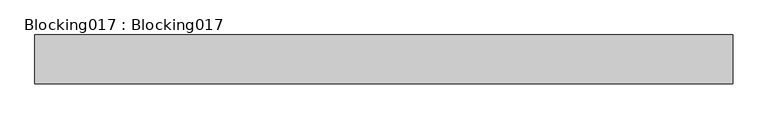
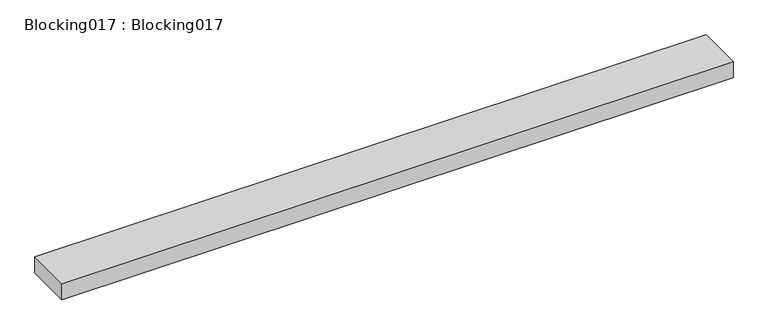
"""IFC4 building model written with IfcOpenShell, lengths in millimetres: proxy geometry, Blocking017 : Blocking017."""

import ifcopenshell
import ifcopenshell.guid

model = None  # the IFC model being written
_history = None  # IfcOwnerHistory: only IFC2X3 demands one
_inside = {}  # id of a spatial element -> (the spatial element, [elements in it])
_under = {}  # id of a project, library or spatial element -> (it, [spatial elements below it])
_declared = {}  # id of a project -> (the project, [libraries it declares])
_typed = {}  # id of a type object -> (the type object, [elements of that type])
_made_of = {}  # id of a material, layer set ... -> (it, [elements and type objects made of it])


def new_model(schema):
    """Start an empty IFC model of exactly this schema.

    Asked for "IFC4X3", IfcOpenShell would pick the latest addendum, in which some entities
    have other attributes; the version numbers below select the first issue.
    IFC2X3 requires an IfcOwnerHistory on every rooted entity: one is made here for all.
    """
    global model, _history
    if schema == "IFC4X3":
        model = ifcopenshell.file(schema_version=(4, 3, 0, 0))
    else:
        model = ifcopenshell.file(schema=schema)
    _inside.clear()
    _under.clear()
    _declared.clear()
    _typed.clear()
    _made_of.clear()
    _history = None
    if model.schema == "IFC2X3":
        org = make("IfcOrganization", Name="unknown")
        user = make(
            "IfcPersonAndOrganization",
            ThePerson=make("IfcPerson", FamilyName="unknown"),
            TheOrganization=org,
        )
        app = make(
            "IfcApplication",
            ApplicationDeveloper=org,
            Version="unknown",
            ApplicationFullName="unknown",
            ApplicationIdentifier="unknown",
        )
        _history = make(
            "IfcOwnerHistory",
            OwningUser=user,
            OwningApplication=app,
            ChangeAction="ADDED",
            CreationDate=0,
        )
    return model


def make(cls, **values):
    """One entity of the class cls with the attributes given. An attribute that is None is left unset."""
    return model.create_entity(
        cls, **{name: value for name, value in values.items() if value is not None}
    )


def rooted(cls, **values):
    """An entity with a GlobalId (a new one), such as an element, a storey or a relation."""
    return make(cls, GlobalId=ifcopenshell.guid.new(), OwnerHistory=_history, **values)


def si_unit(unit_type, name, prefix=None):
    """IfcSIUnit, for example si_unit("LENGTHUNIT", "METRE", prefix="MILLI")."""
    return make("IfcSIUnit", UnitType=unit_type, Prefix=prefix, Name=name)


def assignment(units):
    """IfcUnitAssignment: the units of a project."""
    return None if units is None else make("IfcUnitAssignment", Units=units)


def point(xyz):
    """IfcCartesianPoint."""
    return None if xyz is None else make("IfcCartesianPoint", Coordinates=xyz)


def direction(xyz):
    """IfcDirection."""
    return None if xyz is None else make("IfcDirection", DirectionRatios=xyz)


def frame(location, z_axis=None, x_axis=None):
    """IfcAxis2Placement3D, a coordinate frame: its origin and axes. An axis left out is left unset."""
    return make(
        "IfcAxis2Placement3D",
        Location=point(location),
        Axis=direction(z_axis),
        RefDirection=direction(x_axis),
    )


def origin():
    """The frame at (0, 0, 0) with its axes left unset."""
    return frame((0.0, 0.0, 0.0))


def place(relative_to, where):
    """IfcLocalPlacement: puts the frame where relative to a parent placement (None: the world)."""
    return make(
        "IfcLocalPlacement", PlacementRelTo=relative_to, RelativePlacement=where
    )


def context(
    kind, dimensions, precision=None, world=None, true_north=None, identifier=None
):
    """IfcGeometricRepresentationContext, for example the 3D "Model" context."""
    return make(
        "IfcGeometricRepresentationContext",
        ContextIdentifier=identifier,
        ContextType=kind,
        CoordinateSpaceDimension=dimensions,
        Precision=precision,
        WorldCoordinateSystem=world,
        TrueNorth=true_north,
    )


def project(units=None, contexts=None):
    """IfcProject with its units and contexts."""
    return rooted(
        "IfcProject",
        Name="project",
        RepresentationContexts=contexts,
        UnitsInContext=assignment(units),
    )


def spatial(cls, under=None, at=None, **own):
    """A site, building, storey or space (cls), placed at a placement, below another one or the project."""
    s = rooted(cls, ObjectPlacement=at, **own)
    if under is not None:
        _under.setdefault(under.id(), (under, []))[1].append(s)
    return s


def polyline(points):
    """IfcPolyline through the points."""
    return make("IfcPolyline", Points=[point(p) for p in points])


def outline(outer, holes=None, kind="AREA"):
    """IfcArbitraryClosedProfileDef: a profile drawn as a closed curve; with holes, ...WithVoids."""
    if holes is None:
        return make("IfcArbitraryClosedProfileDef", ProfileType=kind, OuterCurve=outer)
    return make(
        "IfcArbitraryProfileDefWithVoids",
        ProfileType=kind,
        OuterCurve=outer,
        InnerCurves=holes,
    )


def extrude(swept, where, along, depth):
    """IfcExtrudedAreaSolid: the profile swept, set in the frame where, extruded along a direction by depth."""
    return make(
        "IfcExtrudedAreaSolid",
        SweptArea=swept,
        Position=where,
        ExtrudedDirection=direction(along),
        Depth=depth,
    )


def shape(context_of_items, identifier, shape_type, items):
    """IfcShapeRepresentation: the items that make up one representation, for example the "Body"."""
    return make(
        "IfcShapeRepresentation",
        ContextOfItems=context_of_items,
        RepresentationIdentifier=identifier,
        RepresentationType=shape_type,
        Items=items,
    )


def source(mapping_origin, context_of_items, identifier, shape_type, items):
    """IfcRepresentationMap: a shape defined once, which mapped items show again and again."""
    return make(
        "IfcRepresentationMap",
        MappingOrigin=mapping_origin,
        MappedRepresentation=shape(context_of_items, identifier, shape_type, items),
    )


def transform(
    local_origin,
    x_axis=None,
    y_axis=None,
    z_axis=None,
    scale=None,
    scale2=None,
    scale3=None,
    uniform=True,
):
    """IfcCartesianTransformationOperator3D, or its non-uniform kind. x_axis, y_axis, z_axis: its Axis1, 2, 3."""
    if uniform:
        return make(
            "IfcCartesianTransformationOperator3D",
            Axis1=direction(x_axis),
            Axis2=direction(y_axis),
            LocalOrigin=point(local_origin),
            Scale=scale,
            Axis3=direction(z_axis),
        )
    return make(
        "IfcCartesianTransformationOperator3DnonUniform",
        Axis1=direction(x_axis),
        Axis2=direction(y_axis),
        LocalOrigin=point(local_origin),
        Scale=scale,
        Axis3=direction(z_axis),
        Scale2=scale2,
        Scale3=scale3,
    )


def mapped(mapping_source, mapping_target):
    """IfcMappedItem: shows the shape of a source again, moved by a transform."""
    return make(
        "IfcMappedItem", MappingSource=mapping_source, MappingTarget=mapping_target
    )


def made_of(thing, what):
    """Note that an element or type object is made of a material, layer set ...; save() writes the relation."""
    if what is not None:
        _made_of.setdefault(what.id(), (what, []))[1].append(thing)
    return thing


def element(
    cls,
    number,
    at=None,
    inside=None,
    cuts=None,
    type_object=None,
    material=None,
    context=None,
    identifier="Body",
    shape_type=None,
    held_by="IfcProductDefinitionShape",
    body=None,
    shapes=None,
    **own,
):
    """One element of the class cls, such as IfcWall. Its Tag is "e" and its number.

    at: its placement. inside: the storey or other place that contains it. cuts: it is an
    opening in that element (IfcRelVoidsElement). A single representation is given by context,
    identifier, shape_type and body (its items); several are given by shapes. held_by: the class
    of the entity that holds the representations. save() writes the other relations.
    """
    e = rooted(cls, Tag="e%d" % number, ObjectPlacement=at, **own)
    if body is not None:
        shapes = [shape(context, identifier, shape_type, body)]
    if shapes is not None:
        e.Representation = make(held_by, Representations=shapes)
    if inside is not None:
        _inside.setdefault(inside.id(), (inside, []))[1].append(e)
    if cuts is not None:
        rooted(
            "IfcRelVoidsElement", RelatingBuildingElement=cuts, RelatedOpeningElement=e
        )
    if type_object is not None:
        _typed.setdefault(type_object.id(), (type_object, []))[1].append(e)
    return made_of(e, material)


def aggregate(whole, parts):
    """IfcRelAggregates: a whole, such as a stair, and the parts it consists of."""
    return rooted("IfcRelAggregates", RelatingObject=whole, RelatedObjects=parts)


def save(model, path):
    """Write the relations noted so far, then the file.

    IfcRelAggregates (storeys below a building ...), IfcRelContainedInSpatialStructure (elements
    in a storey), IfcRelDefinesByType, IfcRelAssociatesMaterial and IfcRelDeclares: one each for
    every whole, place, type object, material and project.
    """
    for whole, parts in _under.values():
        aggregate(whole, parts)
    for where, things in _inside.values():
        rooted(
            "IfcRelContainedInSpatialStructure",
            RelatedElements=things,
            RelatingStructure=where,
        )
    for kind, things in _typed.values():
        rooted("IfcRelDefinesByType", RelatedObjects=things, RelatingType=kind)
    for what, things in _made_of.values():
        rooted("IfcRelAssociatesMaterial", RelatedObjects=things, RelatingMaterial=what)
    for by, libraries in _declared.values():
        rooted("IfcRelDeclares", RelatingContext=by, RelatedDefinitions=libraries)
    model.write(path)


def blocking017_blocking017_bbcb4067(model_context):
    return source(origin(), model_context, "Body", "SweptSolid", [
        extrude(outline(polyline([(14383.0178845, -4250.1925368), (14383.0178845, -4389.8925368), (12383.0178845, -4389.8925368), (12383.0178845, -4250.1925368), (14383.0178845, -4250.1925368)])), frame((0.0, 0.0, 41004.8787187), z_axis=(0.0, 0.0, 1.0), x_axis=(1.0, 0.0, 0.0)), (0.0, 0.0, 1.0), 50.8),
    ])


if __name__ == "__main__":
    model = new_model("IFC4")
    model_context = context("Model", 3, world=origin())
    ifc_project = project(units=[si_unit("LENGTHUNIT", "METRE", prefix="MILLI")], contexts=[model_context])
    site = spatial("IfcSite", under=ifc_project)
    building = spatial("IfcBuilding", under=site)
    placement = place(None, origin())
    blocking017_blocking017_shape = blocking017_blocking017_bbcb4067(model_context)
    element("IfcBuildingElementProxy", 1, Name="Blocking017 : Blocking017", ObjectType="Blocking017 : Blocking017", at=placement, inside=building, context=model_context, shape_type="MappedRepresentation", body=[
        mapped(blocking017_blocking017_shape, transform((0.0, 0.0, 0.0), x_axis=(1.0, 0.0, 0.0), y_axis=(0.0, 1.0, 0.0), z_axis=(0.0, 0.0, 1.0))),
    ])
    save(model, "model.ifc")

# Revit data of these elements
# Type "Blocking017 : Blocking017"
#   NameOverride = "Blocking017"
# Element 1 (IfcBuildingElementProxy, "Blocking017 : Blocking017")
#   Materials on its faces: "WOOD BLOCKING AS REQUIRED"
# Materials
#   "WOOD BLOCKING AS REQUIRED": class "Unassigned", colour RGB 166 124 85, transparency 0, Cost = 0
